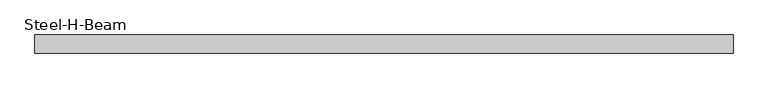
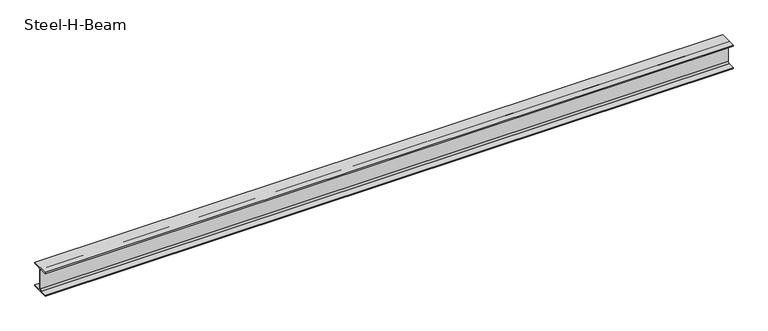
"""IFC4 building model written with IfcOpenShell, lengths in millimetres: beam geometry, Steel-H-Beam : BM121_H-244×175x7x11."""

from ifc_helpers import new_model, si_unit, point, frame, frame_2d, origin, place, context, project, spatial, polyline, circle_curve, trimmed, segment, composite_curve, outline, extrude, source, transform, mapped, element, save


def steel_h_beam_0520d745(model_context):
    return source(origin(), model_context, "Body", "SweptSolid", [
        extrude(outline(composite_curve([segment(polyline([(87.5, -111.0), (87.5, -122.0), (-87.5, -122.0), (-87.5, -111.0), (-19.5, -111.0)]), True, "CONTINUOUS"), segment(trimmed(circle_curve(frame_2d((-19.5, -95.0)), 16.0), [point((-19.5, -111.0))], [point((-3.5, -95.0))], True, "CARTESIAN"), True, "CONTINUOUS"), segment(polyline([(-3.5, -95.0), (-3.5, 95.0)]), True, "CONTINUOUS"), segment(trimmed(circle_curve(frame_2d((-19.5, 95.0)), 16.0), [point((-3.5, 95.0))], [point((-19.5, 111.0))], True, "CARTESIAN"), True, "CONTINUOUS"), segment(polyline([(-19.5, 111.0), (-87.5, 111.0), (-87.5, 122.0), (87.5, 122.0), (87.5, 111.0), (19.5, 111.0)]), True, "CONTINUOUS"), segment(trimmed(circle_curve(frame_2d((19.5, 95.0)), 16.0), [point((19.5, 111.0))], [point((3.5, 95.0))], True, "CARTESIAN"), True, "CONTINUOUS"), segment(polyline([(3.5, 95.0), (3.5, -95.0)]), True, "CONTINUOUS"), segment(trimmed(circle_curve(frame_2d((19.5, -95.0)), 16.0), [point((3.5, -95.0))], [point((19.5, -111.0))], True, "CARTESIAN"), True, "CONTINUOUS"), segment(polyline([(19.5, -111.0), (87.5, -111.0)]), True, "CONTINUOUS")], self_intersect=False)), frame((-3363.2513255, 0.0, 0.0), z_axis=(1.0, 0.0, 0.0), x_axis=(0.0, 1.0, 0.0)), (0.0, 0.0, 1.0), 6724.6),
    ])


if __name__ == "__main__":
    model = new_model("IFC4")
    model_context = context("Model", 3, world=origin())
    ifc_project = project(units=[si_unit("LENGTHUNIT", "METRE", prefix="MILLI")], contexts=[model_context])
    site = spatial("IfcSite", under=ifc_project)
    building = spatial("IfcBuilding", under=site)
    placement = place(None, origin())
    steel_h_beam_shape = steel_h_beam_0520d745(model_context)
    element("IfcBeam", 1, ObjectType="Steel-H-Beam : BM121_H-244×175x7x11", at=placement, inside=building, context=model_context, shape_type="MappedRepresentation", body=[
        mapped(steel_h_beam_shape, transform((0.0, 0.0, 0.0), x_axis=(1.0, 0.0, 0.0), y_axis=(0.0, 1.0, 0.0), z_axis=(0.0, 0.0, 1.0))),
    ])
    save(model, "model.ifc")

# Revit data of these elements
# Type "Steel-H-Beam : BM121_H-244×175x7x11"
#   Surface Area = 1.14653 m²/m
#   Section Area = 56.2375 cm²
#   Mass per Unit Length = 44.1465 kg/m
#   Length [instance default] = 3000 mm
#   B = 175 mm
#   H = 244 mm
#   r = 16 mm
#   tw = 7 mm
#   tf = 11 mm
#   hec_material4 [instance default] = none
#   hec_material3 [instance default] = none
#   hec_material2 [instance default] = none
#   hec_material1 [instance default] = none
#   Structural Material [instance default] = Steel, 45-345
#   Assembly Code = ""
# Element 1 (IfcBeam, "Steel-H-Beam : BM121_H-244×175x7x11")
#   Structural Material = S03AA028-00001_Main Steel Structure Erection Work_Shelter/Building_Medium Steel
#   Materials on its faces: "S03AA028-00001_Main Steel Structure Erection Work_Shelter/Building_Medium Steel"
# Materials
#   "Steel, 45-345": class "Metal", colour RGB 189 187 185, transparency 0, Description = "Steel 345 MPa", Cost = 0
#   "S03AA028-00001_Main Steel Structure Erection Work_Shelter/Building_Medium Steel": class "Metal", colour RGB 120 120 120, transparency 0, Comments = "(90KG/M>Weight≥30KG/M)", Description = "Structural steel 50ksi", W00) Work Master Code = "S03AA028-0001", W01) Work Master_Lv1 = "Main Steel Structure Erection Work", W02) Work Master_Lv2 = "Shelter/Building", W03) Work Master_Spec.1 = "Medium Steel (90KG/M>Weight≥30KG/M)", Cost = 0
